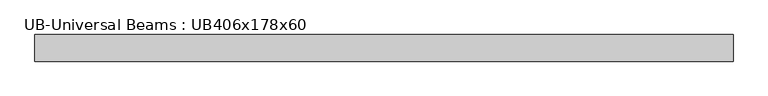
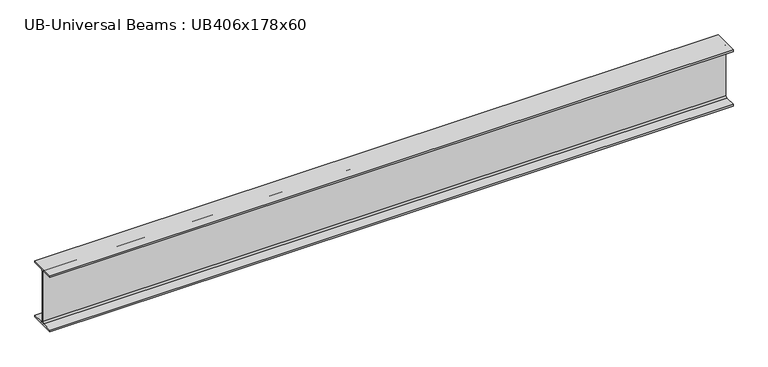
"""IFC4 building model written with IfcOpenShell, lengths in millimetres: beam geometry, UB-Universal Beams : UB406x178x60."""

import ifcopenshell
import ifcopenshell.guid

model = None  # the IFC model being written
_history = None  # IfcOwnerHistory: only IFC2X3 demands one
_inside = {}  # id of a spatial element -> (the spatial element, [elements in it])
_under = {}  # id of a project, library or spatial element -> (it, [spatial elements below it])
_declared = {}  # id of a project -> (the project, [libraries it declares])
_typed = {}  # id of a type object -> (the type object, [elements of that type])
_made_of = {}  # id of a material, layer set ... -> (it, [elements and type objects made of it])


def new_model(schema):
    """Start an empty IFC model of exactly this schema.

    Asked for "IFC4X3", IfcOpenShell would pick the latest addendum, in which some entities
    have other attributes; the version numbers below select the first issue.
    IFC2X3 requires an IfcOwnerHistory on every rooted entity: one is made here for all.
    """
    global model, _history
    if schema == "IFC4X3":
        model = ifcopenshell.file(schema_version=(4, 3, 0, 0))
    else:
        model = ifcopenshell.file(schema=schema)
    _inside.clear()
    _under.clear()
    _declared.clear()
    _typed.clear()
    _made_of.clear()
    _history = None
    if model.schema == "IFC2X3":
        org = make("IfcOrganization", Name="unknown")
        user = make(
            "IfcPersonAndOrganization",
            ThePerson=make("IfcPerson", FamilyName="unknown"),
            TheOrganization=org,
        )
        app = make(
            "IfcApplication",
            ApplicationDeveloper=org,
            Version="unknown",
            ApplicationFullName="unknown",
            ApplicationIdentifier="unknown",
        )
        _history = make(
            "IfcOwnerHistory",
            OwningUser=user,
            OwningApplication=app,
            ChangeAction="ADDED",
            CreationDate=0,
        )
    return model


def make(cls, **values):
    """One entity of the class cls with the attributes given. An attribute that is None is left unset."""
    return model.create_entity(
        cls, **{name: value for name, value in values.items() if value is not None}
    )


def rooted(cls, **values):
    """An entity with a GlobalId (a new one), such as an element, a storey or a relation."""
    return make(cls, GlobalId=ifcopenshell.guid.new(), OwnerHistory=_history, **values)


def si_unit(unit_type, name, prefix=None):
    """IfcSIUnit, for example si_unit("LENGTHUNIT", "METRE", prefix="MILLI")."""
    return make("IfcSIUnit", UnitType=unit_type, Prefix=prefix, Name=name)


def assignment(units):
    """IfcUnitAssignment: the units of a project."""
    return None if units is None else make("IfcUnitAssignment", Units=units)


def point(xyz):
    """IfcCartesianPoint."""
    return None if xyz is None else make("IfcCartesianPoint", Coordinates=xyz)


def direction(xyz):
    """IfcDirection."""
    return None if xyz is None else make("IfcDirection", DirectionRatios=xyz)


def frame(location, z_axis=None, x_axis=None):
    """IfcAxis2Placement3D, a coordinate frame: its origin and axes. An axis left out is left unset."""
    return make(
        "IfcAxis2Placement3D",
        Location=point(location),
        Axis=direction(z_axis),
        RefDirection=direction(x_axis),
    )


def frame_2d(location, x_axis=None):
    """IfcAxis2Placement2D, a coordinate frame in the plane: its origin and x axis."""
    return make(
        "IfcAxis2Placement2D", Location=point(location), RefDirection=direction(x_axis)
    )


def origin():
    """The frame at (0, 0, 0) with its axes left unset."""
    return frame((0.0, 0.0, 0.0))


def place(relative_to, where):
    """IfcLocalPlacement: puts the frame where relative to a parent placement (None: the world)."""
    return make(
        "IfcLocalPlacement", PlacementRelTo=relative_to, RelativePlacement=where
    )


def context(
    kind, dimensions, precision=None, world=None, true_north=None, identifier=None
):
    """IfcGeometricRepresentationContext, for example the 3D "Model" context."""
    return make(
        "IfcGeometricRepresentationContext",
        ContextIdentifier=identifier,
        ContextType=kind,
        CoordinateSpaceDimension=dimensions,
        Precision=precision,
        WorldCoordinateSystem=world,
        TrueNorth=true_north,
    )


def project(units=None, contexts=None):
    """IfcProject with its units and contexts."""
    return rooted(
        "IfcProject",
        Name="project",
        RepresentationContexts=contexts,
        UnitsInContext=assignment(units),
    )


def spatial(cls, under=None, at=None, **own):
    """A site, building, storey or space (cls), placed at a placement, below another one or the project."""
    s = rooted(cls, ObjectPlacement=at, **own)
    if under is not None:
        _under.setdefault(under.id(), (under, []))[1].append(s)
    return s


def polyline(points):
    """IfcPolyline through the points."""
    return make("IfcPolyline", Points=[point(p) for p in points])


def circle_curve(where, radius):
    """IfcCircle in the frame where."""
    return make("IfcCircle", Position=where, Radius=radius)


def trimmed(basis, trim1, trim2, sense, master):
    """IfcTrimmedCurve: the piece of a basis curve between two trims."""
    return make(
        "IfcTrimmedCurve",
        BasisCurve=basis,
        Trim1=trim1,
        Trim2=trim2,
        SenseAgreement=sense,
        MasterRepresentation=master,
    )


def segment(curve, same_sense, transition):
    """IfcCompositeCurveSegment."""
    return make(
        "IfcCompositeCurveSegment",
        Transition=transition,
        SameSense=same_sense,
        ParentCurve=curve,
    )


def composite_curve(segments, self_intersect=None):
    """IfcCompositeCurve: segments joined end to end."""
    return make("IfcCompositeCurve", Segments=segments, SelfIntersect=self_intersect)


def outline(outer, holes=None, kind="AREA"):
    """IfcArbitraryClosedProfileDef: a profile drawn as a closed curve; with holes, ...WithVoids."""
    if holes is None:
        return make("IfcArbitraryClosedProfileDef", ProfileType=kind, OuterCurve=outer)
    return make(
        "IfcArbitraryProfileDefWithVoids",
        ProfileType=kind,
        OuterCurve=outer,
        InnerCurves=holes,
    )


def extrude(swept, where, along, depth):
    """IfcExtrudedAreaSolid: the profile swept, set in the frame where, extruded along a direction by depth."""
    return make(
        "IfcExtrudedAreaSolid",
        SweptArea=swept,
        Position=where,
        ExtrudedDirection=direction(along),
        Depth=depth,
    )


def shape(context_of_items, identifier, shape_type, items):
    """IfcShapeRepresentation: the items that make up one representation, for example the "Body"."""
    return make(
        "IfcShapeRepresentation",
        ContextOfItems=context_of_items,
        RepresentationIdentifier=identifier,
        RepresentationType=shape_type,
        Items=items,
    )


def source(mapping_origin, context_of_items, identifier, shape_type, items):
    """IfcRepresentationMap: a shape defined once, which mapped items show again and again."""
    return make(
        "IfcRepresentationMap",
        MappingOrigin=mapping_origin,
        MappedRepresentation=shape(context_of_items, identifier, shape_type, items),
    )


def transform(
    local_origin,
    x_axis=None,
    y_axis=None,
    z_axis=None,
    scale=None,
    scale2=None,
    scale3=None,
    uniform=True,
):
    """IfcCartesianTransformationOperator3D, or its non-uniform kind. x_axis, y_axis, z_axis: its Axis1, 2, 3."""
    if uniform:
        return make(
            "IfcCartesianTransformationOperator3D",
            Axis1=direction(x_axis),
            Axis2=direction(y_axis),
            LocalOrigin=point(local_origin),
            Scale=scale,
            Axis3=direction(z_axis),
        )
    return make(
        "IfcCartesianTransformationOperator3DnonUniform",
        Axis1=direction(x_axis),
        Axis2=direction(y_axis),
        LocalOrigin=point(local_origin),
        Scale=scale,
        Axis3=direction(z_axis),
        Scale2=scale2,
        Scale3=scale3,
    )


def mapped(mapping_source, mapping_target):
    """IfcMappedItem: shows the shape of a source again, moved by a transform."""
    return make(
        "IfcMappedItem", MappingSource=mapping_source, MappingTarget=mapping_target
    )


def made_of(thing, what):
    """Note that an element or type object is made of a material, layer set ...; save() writes the relation."""
    if what is not None:
        _made_of.setdefault(what.id(), (what, []))[1].append(thing)
    return thing


def element(
    cls,
    number,
    at=None,
    inside=None,
    cuts=None,
    type_object=None,
    material=None,
    context=None,
    identifier="Body",
    shape_type=None,
    held_by="IfcProductDefinitionShape",
    body=None,
    shapes=None,
    **own,
):
    """One element of the class cls, such as IfcWall. Its Tag is "e" and its number.

    at: its placement. inside: the storey or other place that contains it. cuts: it is an
    opening in that element (IfcRelVoidsElement). A single representation is given by context,
    identifier, shape_type and body (its items); several are given by shapes. held_by: the class
    of the entity that holds the representations. save() writes the other relations.
    """
    e = rooted(cls, Tag="e%d" % number, ObjectPlacement=at, **own)
    if body is not None:
        shapes = [shape(context, identifier, shape_type, body)]
    if shapes is not None:
        e.Representation = make(held_by, Representations=shapes)
    if inside is not None:
        _inside.setdefault(inside.id(), (inside, []))[1].append(e)
    if cuts is not None:
        rooted(
            "IfcRelVoidsElement", RelatingBuildingElement=cuts, RelatedOpeningElement=e
        )
    if type_object is not None:
        _typed.setdefault(type_object.id(), (type_object, []))[1].append(e)
    return made_of(e, material)


def aggregate(whole, parts):
    """IfcRelAggregates: a whole, such as a stair, and the parts it consists of."""
    return rooted("IfcRelAggregates", RelatingObject=whole, RelatedObjects=parts)


def save(model, path):
    """Write the relations noted so far, then the file.

    IfcRelAggregates (storeys below a building ...), IfcRelContainedInSpatialStructure (elements
    in a storey), IfcRelDefinesByType, IfcRelAssociatesMaterial and IfcRelDeclares: one each for
    every whole, place, type object, material and project.
    """
    for whole, parts in _under.values():
        aggregate(whole, parts)
    for where, things in _inside.values():
        rooted(
            "IfcRelContainedInSpatialStructure",
            RelatedElements=things,
            RelatingStructure=where,
        )
    for kind, things in _typed.values():
        rooted("IfcRelDefinesByType", RelatedObjects=things, RelatingType=kind)
    for what, things in _made_of.values():
        rooted("IfcRelAssociatesMaterial", RelatedObjects=things, RelatingMaterial=what)
    for by, libraries in _declared.values():
        rooted("IfcRelDeclares", RelatingContext=by, RelatedDefinitions=libraries)
    model.write(path)


def ub_universal_beams_ub406x178x60_425a89a6(model_context):
    return source(origin(), model_context, "Body", "SweptSolid", [
        extrude(outline(composite_curve([segment(polyline([(88.95, -190.4), (88.95, -203.2), (-88.95, -203.2), (-88.95, -190.4), (-14.15, -190.4)]), True, "CONTINUOUS"), segment(trimmed(circle_curve(frame_2d((-14.15, -180.2)), 10.2), [point((-14.15, -190.4))], [point((-3.95, -180.2))], True, "CARTESIAN"), True, "CONTINUOUS"), segment(polyline([(-3.95, -180.2), (-3.95, 180.2)]), True, "CONTINUOUS"), segment(trimmed(circle_curve(frame_2d((-14.15, 180.2)), 10.2), [point((-3.95, 180.2))], [point((-14.15, 190.4))], True, "CARTESIAN"), True, "CONTINUOUS"), segment(polyline([(-14.15, 190.4), (-88.95, 190.4), (-88.95, 203.2), (88.95, 203.2), (88.95, 190.4), (14.15, 190.4)]), True, "CONTINUOUS"), segment(trimmed(circle_curve(frame_2d((14.15, 180.2)), 10.2), [point((14.15, 190.4))], [point((3.95, 180.2))], True, "CARTESIAN"), True, "CONTINUOUS"), segment(polyline([(3.95, 180.2), (3.95, -180.2)]), True, "CONTINUOUS"), segment(trimmed(circle_curve(frame_2d((14.15, -180.2)), 10.2), [point((3.95, -180.2))], [point((14.15, -190.4))], True, "CARTESIAN"), True, "CONTINUOUS"), segment(polyline([(14.15, -190.4), (88.95, -190.4)]), True, "CONTINUOUS")], self_intersect=False)), frame((-2334.6, 0.0, 0.0), z_axis=(1.0, 0.0, 0.0), x_axis=(0.0, 1.0, 0.0)), (0.0, 0.0, 1.0), 4669.2),
    ])


if __name__ == "__main__":
    model = new_model("IFC4")
    model_context = context("Model", 3, world=origin())
    ifc_project = project(units=[si_unit("LENGTHUNIT", "METRE", prefix="MILLI")], contexts=[model_context])
    site = spatial("IfcSite", under=ifc_project)
    building = spatial("IfcBuilding", under=site)
    placement = place(None, origin())
    ub_universal_beams_ub406x178x60_shape = ub_universal_beams_ub406x178x60_425a89a6(model_context)
    element("IfcBeam", 1, ObjectType="UB-Universal Beams : UB406x178x60", at=placement, inside=building, context=model_context, shape_type="MappedRepresentation", body=[
        mapped(ub_universal_beams_ub406x178x60_shape, transform((0.0, 0.0, 0.0), x_axis=(1.0, 0.0, 0.0), y_axis=(0.0, 1.0, 0.0), z_axis=(0.0, 0.0, 1.0))),
    ])
    save(model, "model.ifc")

# Revit data of these elements
# Type "UB-Universal Beams : UB406x178x60"
#   Section Name Key = "UB406X178X60"
#   Width = 17.79 cm
#   Web Thickness = 0.79 cm
#   Web Fillet = 1.02 cm
#   Warping Constant = 466000.0 cm⁶
#   Torsional Moment of Inertia = 33.30 cm⁴
#   Section Area = 76.5 cm²
#   Plastic Modulus weak axis = 209.0 cm³
#   Plastic Modulus strong axis = 1200.0 cm³
#   Nominal Weight = 60.0998 kgf/m
#   Moment of Inertia weak axis = 1203.00 cm⁴
#   Moment of Inertia strong axis = 21596.00 cm⁴
#   Height = 40.64 cm
#   Flange Thickness = 1.28 cm
#   Elastic Modulus weak axis = 135.0 cm³
#   Elastic Modulus strong axis = 1063.0 cm³
#   Centroid Vertical = 20.32 cm
#   Centroid Horizontal = 8.895 cm
#   Bolt Spacing = 9.0 cm
#   Length [instance default] = 1500 mm
#   Structural Material [instance default] = Metal - Steel 43-275
#   Type Comments = ""
#   Assembly Code = ""
# Element 1 (IfcBeam, "UB-Universal Beams : UB406x178x60")
#   Materials on its faces: "Metal - Steel 43-275"
# Materials
#   "Metal - Steel 43-275": class "Metal", colour RGB 247 247 247, transparency 0, Cost = 0
